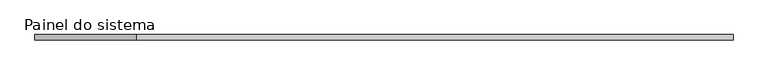
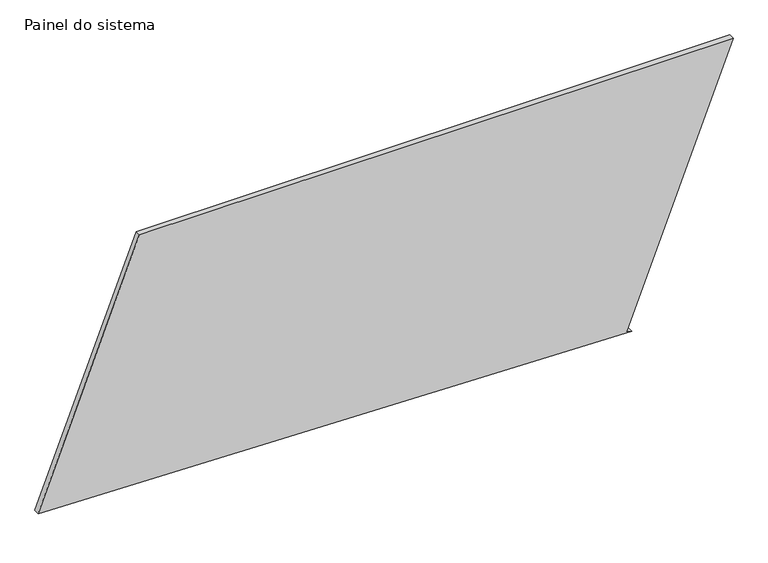
"""IFC4 building model written with IfcOpenShell, lengths in millimetres: plate geometry, Painel do sistema : Envidraçado."""

from ifc_helpers import new_model, si_unit, frame, origin, place, context, project, spatial, polyline, outline, extrude, source, transform, mapped, element, save


def painel_do_sistema_7cd6fada(model_context):
    return source(origin(), model_context, "Body", "SweptSolid", [
        extrude(outline(polyline([(0.0, 1133.8746517), (9.0972802, 1110.5886152), (1264.5469112, 1601.0618295), (1264.5469112, -1134.0847915), (69.2397406, -1601.0618295), (0.0, 1133.8746517)])), frame((0.0, 24.5, 0.0), z_axis=(0.0, 1.0, 0.0), x_axis=(0.0, 0.0, 1.0)), (0.0, 0.0, 1.0), 25.0),
    ])


if __name__ == "__main__":
    model = new_model("IFC4")
    model_context = context("Model", 3, world=origin())
    ifc_project = project(units=[si_unit("LENGTHUNIT", "METRE", prefix="MILLI")], contexts=[model_context])
    site = spatial("IfcSite", under=ifc_project)
    building = spatial("IfcBuilding", under=site)
    placement = place(None, origin())
    painel_do_sistema_shape = painel_do_sistema_7cd6fada(model_context)
    element("IfcPlate", 1, ObjectType="Painel do sistema : Envidraçado", at=placement, inside=building, context=model_context, shape_type="MappedRepresentation", body=[
        mapped(painel_do_sistema_shape, transform((0.0, 0.0, 0.0), x_axis=(1.0, 0.0, 0.0), y_axis=(0.0, 1.0, 0.0), z_axis=(0.0, 0.0, 1.0))),
    ])
    save(model, "model.ifc")

# Revit data of these elements
# Type "Painel do sistema : Envidraçado"
#   Construction Type Id = "GSP4R"
#   Analytic Construction = "Vidraça única Pilkington 1/8 pol"
#   Visual Light Transmittance = 0.9
#   Solar Heat Gain Coefficient = 0.86
#   Heat Transfer Coefficient (U) = 6.7069 W/(m²·K)
# Element 1 (IfcPlate, "Painel do sistema : Envidraçado")
#   Materials on its faces: "Vidro"
# Materials
#   "Vidro": class "Vidro", colour RGB 0 128 192, transparency 0.9, Description = "Vidro de sílica", Cost = 0
